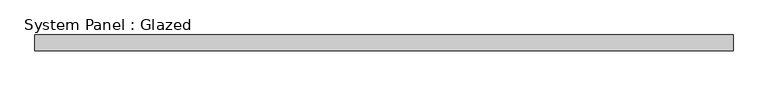
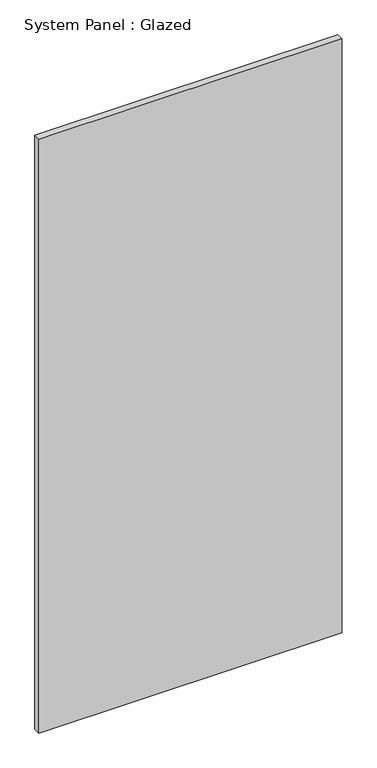
"""IFC4 building model written with IfcOpenShell, lengths in millimetres: plate geometry, System Panel : Glazed."""

import ifcopenshell
import ifcopenshell.guid

model = None  # the IFC model being written
_history = None  # IfcOwnerHistory: only IFC2X3 demands one
_inside = {}  # id of a spatial element -> (the spatial element, [elements in it])
_under = {}  # id of a project, library or spatial element -> (it, [spatial elements below it])
_declared = {}  # id of a project -> (the project, [libraries it declares])
_typed = {}  # id of a type object -> (the type object, [elements of that type])
_made_of = {}  # id of a material, layer set ... -> (it, [elements and type objects made of it])


def new_model(schema):
    """Start an empty IFC model of exactly this schema.

    Asked for "IFC4X3", IfcOpenShell would pick the latest addendum, in which some entities
    have other attributes; the version numbers below select the first issue.
    IFC2X3 requires an IfcOwnerHistory on every rooted entity: one is made here for all.
    """
    global model, _history
    if schema == "IFC4X3":
        model = ifcopenshell.file(schema_version=(4, 3, 0, 0))
    else:
        model = ifcopenshell.file(schema=schema)
    _inside.clear()
    _under.clear()
    _declared.clear()
    _typed.clear()
    _made_of.clear()
    _history = None
    if model.schema == "IFC2X3":
        org = make("IfcOrganization", Name="unknown")
        user = make(
            "IfcPersonAndOrganization",
            ThePerson=make("IfcPerson", FamilyName="unknown"),
            TheOrganization=org,
        )
        app = make(
            "IfcApplication",
            ApplicationDeveloper=org,
            Version="unknown",
            ApplicationFullName="unknown",
            ApplicationIdentifier="unknown",
        )
        _history = make(
            "IfcOwnerHistory",
            OwningUser=user,
            OwningApplication=app,
            ChangeAction="ADDED",
            CreationDate=0,
        )
    return model


def make(cls, **values):
    """One entity of the class cls with the attributes given. An attribute that is None is left unset."""
    return model.create_entity(
        cls, **{name: value for name, value in values.items() if value is not None}
    )


def rooted(cls, **values):
    """An entity with a GlobalId (a new one), such as an element, a storey or a relation."""
    return make(cls, GlobalId=ifcopenshell.guid.new(), OwnerHistory=_history, **values)


def si_unit(unit_type, name, prefix=None):
    """IfcSIUnit, for example si_unit("LENGTHUNIT", "METRE", prefix="MILLI")."""
    return make("IfcSIUnit", UnitType=unit_type, Prefix=prefix, Name=name)


def assignment(units):
    """IfcUnitAssignment: the units of a project."""
    return None if units is None else make("IfcUnitAssignment", Units=units)


def point(xyz):
    """IfcCartesianPoint."""
    return None if xyz is None else make("IfcCartesianPoint", Coordinates=xyz)


def direction(xyz):
    """IfcDirection."""
    return None if xyz is None else make("IfcDirection", DirectionRatios=xyz)


def frame(location, z_axis=None, x_axis=None):
    """IfcAxis2Placement3D, a coordinate frame: its origin and axes. An axis left out is left unset."""
    return make(
        "IfcAxis2Placement3D",
        Location=point(location),
        Axis=direction(z_axis),
        RefDirection=direction(x_axis),
    )


def origin():
    """The frame at (0, 0, 0) with its axes left unset."""
    return frame((0.0, 0.0, 0.0))


def origin_with_axes():
    """The frame at (0, 0, 0) with the z axis (0, 0, 1) and the x axis (1, 0, 0) written out."""
    return frame((0.0, 0.0, 0.0), z_axis=(0.0, 0.0, 1.0), x_axis=(1.0, 0.0, 0.0))


def place(relative_to, where):
    """IfcLocalPlacement: puts the frame where relative to a parent placement (None: the world)."""
    return make(
        "IfcLocalPlacement", PlacementRelTo=relative_to, RelativePlacement=where
    )


def context(
    kind, dimensions, precision=None, world=None, true_north=None, identifier=None
):
    """IfcGeometricRepresentationContext, for example the 3D "Model" context."""
    return make(
        "IfcGeometricRepresentationContext",
        ContextIdentifier=identifier,
        ContextType=kind,
        CoordinateSpaceDimension=dimensions,
        Precision=precision,
        WorldCoordinateSystem=world,
        TrueNorth=true_north,
    )


def project(units=None, contexts=None):
    """IfcProject with its units and contexts."""
    return rooted(
        "IfcProject",
        Name="project",
        RepresentationContexts=contexts,
        UnitsInContext=assignment(units),
    )


def spatial(cls, under=None, at=None, **own):
    """A site, building, storey or space (cls), placed at a placement, below another one or the project."""
    s = rooted(cls, ObjectPlacement=at, **own)
    if under is not None:
        _under.setdefault(under.id(), (under, []))[1].append(s)
    return s


def polyline(points):
    """IfcPolyline through the points."""
    return make("IfcPolyline", Points=[point(p) for p in points])


def outline(outer, holes=None, kind="AREA"):
    """IfcArbitraryClosedProfileDef: a profile drawn as a closed curve; with holes, ...WithVoids."""
    if holes is None:
        return make("IfcArbitraryClosedProfileDef", ProfileType=kind, OuterCurve=outer)
    return make(
        "IfcArbitraryProfileDefWithVoids",
        ProfileType=kind,
        OuterCurve=outer,
        InnerCurves=holes,
    )


def extrude(swept, where, along, depth):
    """IfcExtrudedAreaSolid: the profile swept, set in the frame where, extruded along a direction by depth."""
    return make(
        "IfcExtrudedAreaSolid",
        SweptArea=swept,
        Position=where,
        ExtrudedDirection=direction(along),
        Depth=depth,
    )


def shape(context_of_items, identifier, shape_type, items):
    """IfcShapeRepresentation: the items that make up one representation, for example the "Body"."""
    return make(
        "IfcShapeRepresentation",
        ContextOfItems=context_of_items,
        RepresentationIdentifier=identifier,
        RepresentationType=shape_type,
        Items=items,
    )


def source(mapping_origin, context_of_items, identifier, shape_type, items):
    """IfcRepresentationMap: a shape defined once, which mapped items show again and again."""
    return make(
        "IfcRepresentationMap",
        MappingOrigin=mapping_origin,
        MappedRepresentation=shape(context_of_items, identifier, shape_type, items),
    )


def transform(
    local_origin,
    x_axis=None,
    y_axis=None,
    z_axis=None,
    scale=None,
    scale2=None,
    scale3=None,
    uniform=True,
):
    """IfcCartesianTransformationOperator3D, or its non-uniform kind. x_axis, y_axis, z_axis: its Axis1, 2, 3."""
    if uniform:
        return make(
            "IfcCartesianTransformationOperator3D",
            Axis1=direction(x_axis),
            Axis2=direction(y_axis),
            LocalOrigin=point(local_origin),
            Scale=scale,
            Axis3=direction(z_axis),
        )
    return make(
        "IfcCartesianTransformationOperator3DnonUniform",
        Axis1=direction(x_axis),
        Axis2=direction(y_axis),
        LocalOrigin=point(local_origin),
        Scale=scale,
        Axis3=direction(z_axis),
        Scale2=scale2,
        Scale3=scale3,
    )


def mapped(mapping_source, mapping_target):
    """IfcMappedItem: shows the shape of a source again, moved by a transform."""
    return make(
        "IfcMappedItem", MappingSource=mapping_source, MappingTarget=mapping_target
    )


def made_of(thing, what):
    """Note that an element or type object is made of a material, layer set ...; save() writes the relation."""
    if what is not None:
        _made_of.setdefault(what.id(), (what, []))[1].append(thing)
    return thing


def element(
    cls,
    number,
    at=None,
    inside=None,
    cuts=None,
    type_object=None,
    material=None,
    context=None,
    identifier="Body",
    shape_type=None,
    held_by="IfcProductDefinitionShape",
    body=None,
    shapes=None,
    **own,
):
    """One element of the class cls, such as IfcWall. Its Tag is "e" and its number.

    at: its placement. inside: the storey or other place that contains it. cuts: it is an
    opening in that element (IfcRelVoidsElement). A single representation is given by context,
    identifier, shape_type and body (its items); several are given by shapes. held_by: the class
    of the entity that holds the representations. save() writes the other relations.
    """
    e = rooted(cls, Tag="e%d" % number, ObjectPlacement=at, **own)
    if body is not None:
        shapes = [shape(context, identifier, shape_type, body)]
    if shapes is not None:
        e.Representation = make(held_by, Representations=shapes)
    if inside is not None:
        _inside.setdefault(inside.id(), (inside, []))[1].append(e)
    if cuts is not None:
        rooted(
            "IfcRelVoidsElement", RelatingBuildingElement=cuts, RelatedOpeningElement=e
        )
    if type_object is not None:
        _typed.setdefault(type_object.id(), (type_object, []))[1].append(e)
    return made_of(e, material)


def aggregate(whole, parts):
    """IfcRelAggregates: a whole, such as a stair, and the parts it consists of."""
    return rooted("IfcRelAggregates", RelatingObject=whole, RelatedObjects=parts)


def save(model, path):
    """Write the relations noted so far, then the file.

    IfcRelAggregates (storeys below a building ...), IfcRelContainedInSpatialStructure (elements
    in a storey), IfcRelDefinesByType, IfcRelAssociatesMaterial and IfcRelDeclares: one each for
    every whole, place, type object, material and project.
    """
    for whole, parts in _under.values():
        aggregate(whole, parts)
    for where, things in _inside.values():
        rooted(
            "IfcRelContainedInSpatialStructure",
            RelatedElements=things,
            RelatingStructure=where,
        )
    for kind, things in _typed.values():
        rooted("IfcRelDefinesByType", RelatedObjects=things, RelatingType=kind)
    for what, things in _made_of.values():
        rooted("IfcRelAssociatesMaterial", RelatedObjects=things, RelatingMaterial=what)
    for by, libraries in _declared.values():
        rooted("IfcRelDeclares", RelatingContext=by, RelatedDefinitions=libraries)
    model.write(path)


def system_panel_glazed_a5fae1e5(model_context):
    return source(origin(), model_context, "Body", "SweptSolid", [
        extrude(outline(polyline([(565.15, 19.05), (-565.15, 19.05), (-565.15, 44.45), (565.15, 44.45), (565.15, 19.05)])), origin_with_axes(), (0.0, 0.0, 1.0), 2343.15),
    ])


if __name__ == "__main__":
    model = new_model("IFC4")
    model_context = context("Model", 3, world=origin())
    ifc_project = project(units=[si_unit("LENGTHUNIT", "METRE", prefix="MILLI")], contexts=[model_context])
    site = spatial("IfcSite", under=ifc_project)
    building = spatial("IfcBuilding", under=site)
    placement = place(None, origin())
    system_panel_glazed_shape = system_panel_glazed_a5fae1e5(model_context)
    element("IfcPlate", 1, ObjectType="System Panel : Glazed", at=placement, inside=building, context=model_context, shape_type="MappedRepresentation", body=[
        mapped(system_panel_glazed_shape, transform((0.0, 0.0, 0.0), x_axis=(1.0, 0.0, 0.0), y_axis=(0.0, 1.0, 0.0), z_axis=(0.0, 0.0, 1.0))),
    ])
    save(model, "model.ifc")

# Revit data of these elements
# Element 1 (IfcPlate, "System Panel : Glazed")
#   Materials on its faces: "Glass"
# Materials
#   "Glass": class "Glass", colour RGB 0 128 192, transparency 0.75
